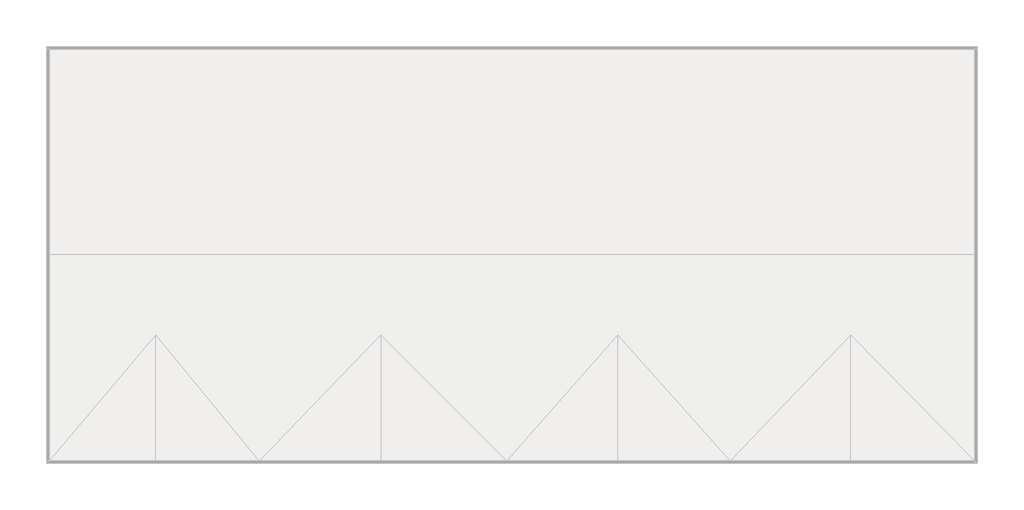
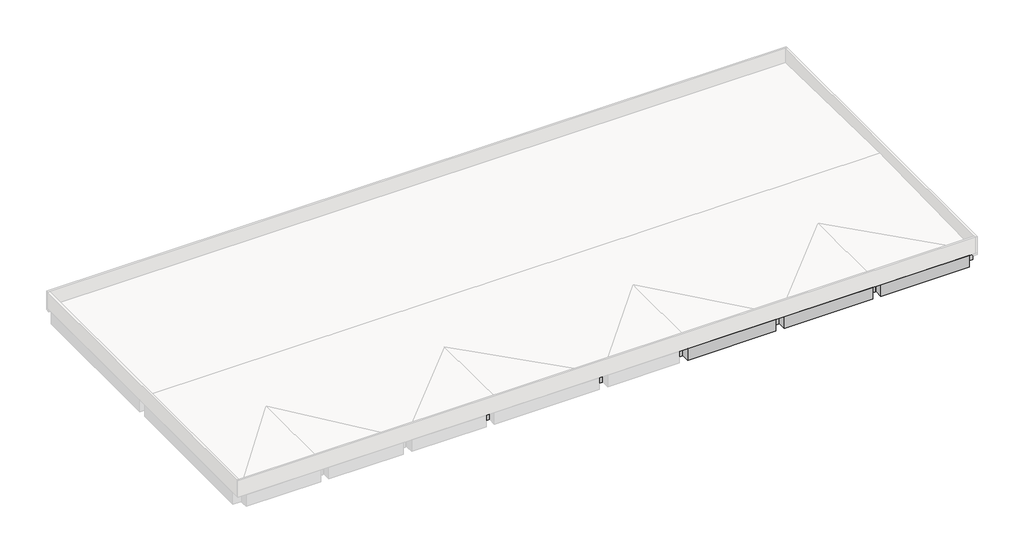
# One storey, part 2 of 2: 43 beams.
"""IFC4 building model written with IfcOpenShell, lengths in millimetres."""

import ifcopenshell
import ifcopenshell.guid

model = None  # the IFC model being written
_history = None  # IfcOwnerHistory: only IFC2X3 demands one
_inside = {}  # id of a spatial element -> (the spatial element, [elements in it])
_under = {}  # id of a project, library or spatial element -> (it, [spatial elements below it])
_declared = {}  # id of a project -> (the project, [libraries it declares])
_typed = {}  # id of a type object -> (the type object, [elements of that type])
_made_of = {}  # id of a material, layer set ... -> (it, [elements and type objects made of it])


def new_model(schema):
    """Start an empty IFC model of exactly this schema.

    Asked for "IFC4X3", IfcOpenShell would pick the latest addendum, in which some entities
    have other attributes; the version numbers below select the first issue.
    IFC2X3 requires an IfcOwnerHistory on every rooted entity: one is made here for all.
    """
    global model, _history
    if schema == "IFC4X3":
        model = ifcopenshell.file(schema_version=(4, 3, 0, 0))
    else:
        model = ifcopenshell.file(schema=schema)
    _inside.clear()
    _under.clear()
    _declared.clear()
    _typed.clear()
    _made_of.clear()
    _history = None
    if model.schema == "IFC2X3":
        org = make("IfcOrganization", Name="unknown")
        user = make(
            "IfcPersonAndOrganization",
            ThePerson=make("IfcPerson", FamilyName="unknown"),
            TheOrganization=org,
        )
        app = make(
            "IfcApplication",
            ApplicationDeveloper=org,
            Version="unknown",
            ApplicationFullName="unknown",
            ApplicationIdentifier="unknown",
        )
        _history = make(
            "IfcOwnerHistory",
            OwningUser=user,
            OwningApplication=app,
            ChangeAction="ADDED",
            CreationDate=0,
        )
    return model


def make(cls, **values):
    """One entity of the class cls with the attributes given. An attribute that is None is left unset."""
    return model.create_entity(
        cls, **{name: value for name, value in values.items() if value is not None}
    )


def rooted(cls, **values):
    """An entity with a GlobalId (a new one), such as an element, a storey or a relation."""
    return make(cls, GlobalId=ifcopenshell.guid.new(), OwnerHistory=_history, **values)


def si_unit(unit_type, name, prefix=None):
    """IfcSIUnit, for example si_unit("LENGTHUNIT", "METRE", prefix="MILLI")."""
    return make("IfcSIUnit", UnitType=unit_type, Prefix=prefix, Name=name)


def assignment(units):
    """IfcUnitAssignment: the units of a project."""
    return None if units is None else make("IfcUnitAssignment", Units=units)


def point(xyz):
    """IfcCartesianPoint."""
    return None if xyz is None else make("IfcCartesianPoint", Coordinates=xyz)


def direction(xyz):
    """IfcDirection."""
    return None if xyz is None else make("IfcDirection", DirectionRatios=xyz)


def frame(location, z_axis=None, x_axis=None):
    """IfcAxis2Placement3D, a coordinate frame: its origin and axes. An axis left out is left unset."""
    return make(
        "IfcAxis2Placement3D",
        Location=point(location),
        Axis=direction(z_axis),
        RefDirection=direction(x_axis),
    )


def origin():
    """The frame at (0, 0, 0) with its axes left unset."""
    return frame((0.0, 0.0, 0.0))


def place(relative_to, where):
    """IfcLocalPlacement: puts the frame where relative to a parent placement (None: the world)."""
    return make(
        "IfcLocalPlacement", PlacementRelTo=relative_to, RelativePlacement=where
    )


def context(
    kind, dimensions, precision=None, world=None, true_north=None, identifier=None
):
    """IfcGeometricRepresentationContext, for example the 3D "Model" context."""
    return make(
        "IfcGeometricRepresentationContext",
        ContextIdentifier=identifier,
        ContextType=kind,
        CoordinateSpaceDimension=dimensions,
        Precision=precision,
        WorldCoordinateSystem=world,
        TrueNorth=true_north,
    )


def project(units=None, contexts=None):
    """IfcProject with its units and contexts."""
    return rooted(
        "IfcProject",
        Name="project",
        RepresentationContexts=contexts,
        UnitsInContext=assignment(units),
    )


def spatial(cls, under=None, at=None, **own):
    """A site, building, storey or space (cls), placed at a placement, below another one or the project."""
    s = rooted(cls, ObjectPlacement=at, **own)
    if under is not None:
        _under.setdefault(under.id(), (under, []))[1].append(s)
    return s


def faces_of(points, faces, orient=None, outer=None):
    """IfcFace entities. A face is a list of loops; a loop is a list of indices into points, from 0.

    orient and outer hold one flag for each loop. By default every Orientation is true, the
    first loop of a face is its IfcFaceOuterBound and the others are IfcFaceBound.
    """
    made = []
    for i, loops in enumerate(faces):
        bounds = []
        for j, loop in enumerate(loops):
            is_outer = j == 0 if outer is None else outer[i][j]
            bounds.append(
                make(
                    "IfcFaceOuterBound" if is_outer else "IfcFaceBound",
                    Bound=make("IfcPolyLoop", Polygon=[points[k] for k in loop]),
                    Orientation=True if orient is None else orient[i][j],
                )
            )
        made.append(make("IfcFace", Bounds=bounds))
    return made


def faceted_brep(points, faces, orient=None, outer=None, voids=None):
    """IfcFacetedBrep: a solid bounded by flat faces; with voids (closed shells), ...WithVoids."""
    shared = [point(p) for p in points]
    hull = make("IfcClosedShell", CfsFaces=faces_of(shared, faces, orient, outer))
    if voids is None:
        return make("IfcFacetedBrep", Outer=hull)
    return make(
        "IfcFacetedBrepWithVoids",
        Outer=hull,
        Voids=[
            make(cls, CfsFaces=faces_of(shared, fs, o, b)) for cls, fs, o, b in voids
        ],
    )


def shape(context_of_items, identifier, shape_type, items):
    """IfcShapeRepresentation: the items that make up one representation, for example the "Body"."""
    return make(
        "IfcShapeRepresentation",
        ContextOfItems=context_of_items,
        RepresentationIdentifier=identifier,
        RepresentationType=shape_type,
        Items=items,
    )


def made_of(thing, what):
    """Note that an element or type object is made of a material, layer set ...; save() writes the relation."""
    if what is not None:
        _made_of.setdefault(what.id(), (what, []))[1].append(thing)
    return thing


def element(
    cls,
    number,
    at=None,
    inside=None,
    cuts=None,
    type_object=None,
    material=None,
    context=None,
    identifier="Body",
    shape_type=None,
    held_by="IfcProductDefinitionShape",
    body=None,
    shapes=None,
    **own,
):
    """One element of the class cls, such as IfcWall. Its Tag is "e" and its number.

    at: its placement. inside: the storey or other place that contains it. cuts: it is an
    opening in that element (IfcRelVoidsElement). A single representation is given by context,
    identifier, shape_type and body (its items); several are given by shapes. held_by: the class
    of the entity that holds the representations. save() writes the other relations.
    """
    e = rooted(cls, Tag="e%d" % number, ObjectPlacement=at, **own)
    if body is not None:
        shapes = [shape(context, identifier, shape_type, body)]
    if shapes is not None:
        e.Representation = make(held_by, Representations=shapes)
    if inside is not None:
        _inside.setdefault(inside.id(), (inside, []))[1].append(e)
    if cuts is not None:
        rooted(
            "IfcRelVoidsElement", RelatingBuildingElement=cuts, RelatedOpeningElement=e
        )
    if type_object is not None:
        _typed.setdefault(type_object.id(), (type_object, []))[1].append(e)
    return made_of(e, material)


def aggregate(whole, parts):
    """IfcRelAggregates: a whole, such as a stair, and the parts it consists of."""
    return rooted("IfcRelAggregates", RelatingObject=whole, RelatedObjects=parts)


def save(model, path):
    """Write the relations noted so far, then the file.

    IfcRelAggregates (storeys below a building ...), IfcRelContainedInSpatialStructure (elements
    in a storey), IfcRelDefinesByType, IfcRelAssociatesMaterial and IfcRelDeclares: one each for
    every whole, place, type object, material and project.
    """
    for whole, parts in _under.values():
        aggregate(whole, parts)
    for where, things in _inside.values():
        rooted(
            "IfcRelContainedInSpatialStructure",
            RelatedElements=things,
            RelatingStructure=where,
        )
    for kind, things in _typed.values():
        rooted("IfcRelDefinesByType", RelatedObjects=things, RelatingType=kind)
    for what, things in _made_of.values():
        rooted("IfcRelAssociatesMaterial", RelatedObjects=things, RelatingMaterial=what)
    for by, libraries in _declared.values():
        rooted("IfcRelDeclares", RelatingContext=by, RelatedDefinitions=libraries)
    model.write(path)


model = new_model("IFC4")

# Units and contexts
model_context = context("Model", 3, world=origin())
ifc_project = project(units=[si_unit("LENGTHUNIT", "METRE", prefix="MILLI")], contexts=[model_context])

# Site, building, storey
site = spatial("IfcSite", under=ifc_project)
building = spatial("IfcBuilding", under=site)
storey = spatial("IfcBuildingStorey", under=building, Name="TOC", Elevation=104550.0)

# Beams
placement = place(None, origin())
element("IfcBeam", 1, ObjectType="RC Beam_Rectangular : H_SB_AR S16_RC Beam-AG_600x900_RG9", at=placement, inside=storey, context=model_context, shape_type="Brep", body=[
    faceted_brep([(300.0, 4200.0, 104550.0), (300.0, 3600.0, 104550.0), (2800.0, 3600.0, 104550.0), (3200.0, 3600.0, 104550.0), (5700.0, 3600.0, 104550.0), (5700.0, 4200.0, 104550.0), (300.0, 3600.0, 104400.0), (300.0, 3600.0, 103650.0), (2800.0, 3600.0, 103650.0), (3200.0, 3600.0, 103650.0), (5700.0, 3600.0, 103650.0), (300.0, 4200.0, 103650.0), (5700.0, 4200.0, 103650.0)], [[[0, 1, 2, 3, 4, 5]], [[1, 6, 7, 8, 9, 10, 4, 3, 2]], [[7, 11, 12, 10, 9, 8]], [[11, 0, 5, 12]], [[1, 0, 11, 7, 6]], [[5, 4, 10, 12]]]),
])
element("IfcBeam", 2, ObjectType="RC Beam_Rectangular : H_SB_AR S16_RC Beam-AG_600x900_RG9", at=placement, inside=storey, context=model_context, shape_type="Brep", body=[
    faceted_brep([(6300.0, 4200.0, 104550.0), (6300.0, 3600.0, 104550.0), (8800.0, 3600.0, 104550.0), (9200.0, 3600.0, 104550.0), (11700.0, 3600.0, 104550.0), (11700.0, 4200.0, 104550.0), (6300.0, 3600.0, 103650.0), (8800.0, 3600.0, 103650.0), (9200.0, 3600.0, 103650.0), (11700.0, 3600.0, 103650.0), (6300.0, 4200.0, 103650.0), (11700.0, 4200.0, 103650.0)], [[[0, 1, 2, 3, 4, 5]], [[1, 6, 7, 8, 9, 4, 3, 2]], [[6, 10, 11, 9, 8, 7]], [[10, 0, 5, 11]], [[1, 0, 10, 6]], [[5, 4, 9, 11]]]),
])
element("IfcBeam", 3, ObjectType="RC Beam_Rectangular : H_SB_AR S16_RC Beam-AG_600x900_RG9", at=placement, inside=storey, context=model_context, shape_type="Brep", body=[
    faceted_brep([(12300.0, 4200.0, 104550.0), (12300.0, 3600.0, 104550.0), (14800.0, 3600.0, 104550.0), (15200.0, 3600.0, 104550.0), (17700.0, 3600.0, 104550.0), (17700.0, 4200.0, 104550.0), (12300.0, 3600.0, 103650.0), (14800.0, 3600.0, 103650.0), (15200.0, 3600.0, 103650.0), (17700.0, 3600.0, 103650.0), (17700.0, 3600.0, 104400.0), (12300.0, 4200.0, 103650.0), (17700.0, 4200.0, 103650.0)], [[[0, 1, 2, 3, 4, 5]], [[1, 6, 7, 8, 9, 10, 4, 3, 2]], [[6, 11, 12, 9, 8, 7]], [[11, 0, 5, 12]], [[1, 0, 11, 6]], [[5, 4, 10, 9, 12]]]),
])
element("IfcBeam", 4, ObjectType="RC Beam_Rectangular : H_SB_AR S16_RC Beam-AG_600x900_RG9", at=placement, inside=storey, context=model_context, shape_type="Brep", body=[
    faceted_brep([(18300.0, 4200.0, 104550.0), (18300.0, 3600.0, 104550.0), (21800.0, 3600.0, 104550.0), (22400.0, 3600.0, 104550.0), (25900.0, 3600.0, 104550.0), (25900.0, 4200.0, 104550.0), (18300.0, 3600.0, 104400.0), (18300.0, 3600.0, 103650.0), (21800.0, 3600.0, 103650.0), (22400.0, 3600.0, 103650.0), (25900.0, 3600.0, 103650.0), (18300.0, 4200.0, 103650.0), (25900.0, 4200.0, 103650.0)], [[[0, 1, 2, 3, 4, 5]], [[1, 6, 7, 8, 9, 10, 4, 3, 2]], [[7, 11, 12, 10, 9, 8]], [[11, 0, 5, 12]], [[7, 6, 1, 0, 11]], [[5, 4, 10, 12]]]),
])
element("IfcBeam", 5, ObjectType="RC Beam_Rectangular : H_SB_AR S16_RC Beam-AG_600x900_RG9", at=placement, inside=storey, context=model_context, shape_type="Brep", body=[
    faceted_brep([(31700.0, 3600.0, 104550.0), (31700.0, 4200.0, 104550.0), (26500.0, 4200.0, 104550.0), (26500.0, 3600.0, 104550.0), (28800.0, 3600.0, 104550.0), (29400.0, 3600.0, 104550.0), (31700.0, 3600.0, 103650.0), (26500.0, 3600.0, 103650.0), (28800.0, 3600.0, 103650.0), (29400.0, 3600.0, 103650.0), (31700.0, 4200.0, 103650.0), (26500.0, 4200.0, 103650.0)], [[[0, 1, 2, 3, 4, 5]], [[6, 0, 5, 4, 3, 7, 8, 9]], [[10, 6, 9, 8, 7, 11]], [[1, 10, 11, 2]], [[1, 0, 6, 10]], [[3, 2, 11, 7]]]),
])
element("IfcBeam", 6, ObjectType="RC Beam_Rectangular : H_SB_AR S16_RC Beam-AG_600x900_RG9", at=placement, inside=storey, context=model_context, shape_type="Brep", body=[
    faceted_brep([(38700.0, 3600.0, 104550.0), (38700.0, 4200.0, 104550.0), (32300.0, 4200.0, 104550.0), (32300.0, 3600.0, 104550.0), (35200.0, 3600.0, 104550.0), (35800.0, 3600.0, 104550.0), (38700.0, 3600.0, 103650.0), (32300.0, 3600.0, 103650.0), (35200.0, 3600.0, 103650.0), (35800.0, 3600.0, 103650.0), (38700.0, 4200.0, 103650.0), (32300.0, 4200.0, 103650.0)], [[[0, 1, 2, 3, 4, 5]], [[6, 0, 5, 4, 3, 7, 8, 9]], [[10, 6, 9, 8, 7, 11]], [[1, 10, 11, 2]], [[1, 0, 6, 10]], [[3, 2, 11, 7]]]),
])
element("IfcBeam", 7, ObjectType="RC Beam_Rectangular : H_SB_AR S16_RC Beam-AG_600x900_RG9", at=placement, inside=storey, context=model_context, shape_type="Brep", body=[
    faceted_brep([(45700.0, 3600.0, 104550.0), (45700.0, 4200.0, 104550.0), (39300.0, 4200.0, 104550.0), (39300.0, 3600.0, 104550.0), (42200.0, 3600.0, 104550.0), (42800.0, 3600.0, 104550.0), (45700.0, 3600.0, 103650.0), (39300.0, 3600.0, 103650.0), (42200.0, 3600.0, 103650.0), (42800.0, 3600.0, 103650.0), (45700.0, 4200.0, 103650.0), (39300.0, 4200.0, 103650.0)], [[[0, 1, 2, 3, 4, 5]], [[6, 0, 5, 4, 3, 7, 8, 9]], [[10, 6, 9, 8, 7, 11]], [[1, 10, 11, 2]], [[1, 0, 6, 10]], [[3, 2, 11, 7]]]),
])
element("IfcBeam", 8, ObjectType="RC Beam_Rectangular : H_SB_AR S16_RC Beam-AG_600x900_RG9", at=placement, inside=storey, context=model_context, shape_type="Brep", body=[
    faceted_brep([(52700.0, 3600.0, 104550.0), (52700.0, 4200.0, 104550.0), (46300.0, 4200.0, 104550.0), (46300.0, 3600.0, 104550.0), (46600.0, 3600.0, 104550.0), (47200.0, 3600.0, 104550.0), (52700.0, 3600.0, 103650.0), (52700.0, 3600.0, 104400.0), (46300.0, 3600.0, 103650.0), (46600.0, 3600.0, 103650.0), (47200.0, 3600.0, 103650.0), (52700.0, 4200.0, 103650.0), (46300.0, 4200.0, 103650.0)], [[[0, 1, 2, 3, 4, 5]], [[6, 7, 0, 5, 4, 3, 8, 9, 10]], [[11, 6, 10, 9, 8, 12]], [[1, 11, 12, 2]], [[1, 0, 7, 6, 11]], [[3, 2, 12, 8]]]),
])
element("IfcBeam", 9, ObjectType="RC Beam_Rectangular : H_SB_AR S16_RC Beam-AG_600x900_RG9", at=placement, inside=storey, context=model_context, shape_type="Brep", body=[
    faceted_brep([(32300.0, -19200.0, 104550.0), (32300.0, -19800.0, 104550.0), (38700.0, -19800.0, 104550.0), (38700.0, -19200.0, 104550.0), (35800.0, -19200.0, 104550.0), (35200.0, -19200.0, 104550.0), (32300.0, -19800.0, 103650.0), (38700.0, -19800.0, 103650.0), (32300.0, -19200.0, 103650.0), (35200.0, -19200.0, 103650.0), (35800.0, -19200.0, 103650.0), (38700.0, -19200.0, 103650.0)], [[[0, 1, 2, 3, 4, 5]], [[1, 6, 7, 2]], [[6, 8, 9, 10, 11, 7]], [[8, 0, 5, 4, 3, 11, 10, 9]], [[1, 0, 8, 6]], [[3, 2, 7, 11]]]),
])
element("IfcBeam", 10, ObjectType="RC Beam_Rectangular : H_SB_AR S16_RC Beam-AG_600x900_RG9", at=placement, inside=storey, context=model_context, shape_type="Brep", body=[
    faceted_brep([(39300.0, -19200.0, 104550.0), (39300.0, -19800.0, 104550.0), (45700.0, -19800.0, 104550.0), (45700.0, -19200.0, 104550.0), (42800.0, -19200.0, 104550.0), (42200.0, -19200.0, 104550.0), (39300.0, -19800.0, 103650.0), (45700.0, -19800.0, 103650.0), (39300.0, -19200.0, 103650.0), (42200.0, -19200.0, 103650.0), (42800.0, -19200.0, 103650.0), (45700.0, -19200.0, 103650.0)], [[[0, 1, 2, 3, 4, 5]], [[1, 6, 7, 2]], [[6, 8, 9, 10, 11, 7]], [[8, 0, 5, 4, 3, 11, 10, 9]], [[1, 0, 8, 6]], [[3, 2, 7, 11]]]),
])
element("IfcBeam", 11, ObjectType="RC Beam_Rectangular : H_SB_AR S16_RC Beam-AG_600x900_RG9", at=placement, inside=storey, context=model_context, shape_type="Brep", body=[
    faceted_brep([(46300.0, -19200.0, 104550.0), (46300.0, -19800.0, 104550.0), (52700.0, -19800.0, 104550.0), (52700.0, -19200.0, 104550.0), (49800.0, -19200.0, 104550.0), (49200.0, -19200.0, 104550.0), (46300.0, -19800.0, 103650.0), (52700.0, -19800.0, 103650.0), (46300.0, -19200.0, 103650.0), (49200.0, -19200.0, 103650.0), (49800.0, -19200.0, 103650.0), (52700.0, -19200.0, 103650.0), (52700.0, -19350.0, 103650.0), (52700.0, -19200.0, 104400.0)], [[[0, 1, 2, 3, 4, 5]], [[1, 6, 7, 2]], [[6, 8, 9, 10, 11, 12, 7]], [[8, 0, 5, 4, 3, 13, 11, 10, 9]], [[1, 0, 8, 6]], [[3, 2, 7, 12, 11, 13]]]),
])
element("IfcBeam", 12, ObjectType="RC Beam_Rectangular : H_SB_AR S16_RC Beam-AG_600x900_RG7", at=placement, inside=storey, context=model_context, shape_type="Brep", body=[
    faceted_brep([(53300.0, 3600.0, 104550.0), (52700.0, 3600.0, 104550.0), (52700.0, -11400.0, 104550.0), (53300.0, -11400.0, 104550.0), (52700.0, 3600.0, 104400.0), (52700.0, 3600.0, 103650.0), (52700.0, -11400.0, 103650.0), (52700.0, -11400.0, 104400.0), (52850.0, 3600.0, 103650.0), (53300.0, 3600.0, 103650.0), (53300.0, -11400.0, 103650.0)], [[[0, 1, 2, 3]], [[1, 4, 5, 6, 7, 2]], [[5, 8, 9, 10, 6]], [[3, 10, 9, 0]], [[0, 9, 8, 5, 4, 1]], [[3, 2, 7, 6, 10]]]),
])
element("IfcBeam", 13, ObjectType="RC Beam_Rectangular : H_SB_AR S16_RC Beam-AG_600x900_RG8", at=placement, inside=storey, context=model_context, shape_type="Brep", body=[
    faceted_brep([(53300.0, -12000.0, 104550.0), (52700.0, -12000.0, 104550.0), (52700.0, -19200.0, 104550.0), (53300.0, -19200.0, 104550.0), (52700.0, -19200.0, 103650.0), (52700.0, -19200.0, 104400.0), (52700.0, -12000.0, 104400.0), (52700.0, -12000.0, 103650.0), (53300.0, -19200.0, 103650.0), (53300.0, -12000.0, 103650.0)], [[[0, 1, 2, 3]], [[4, 5, 2, 1, 6, 7]], [[8, 4, 7, 9]], [[3, 8, 9, 0]], [[2, 5, 4, 8, 3]], [[0, 9, 7, 6, 1]]]),
])
element("IfcBeam", 14, ObjectType="RC Beam_Rectangular : H_SB_AR S16_RC Beam-AG_600x900_RG5", at=placement, inside=storey, context=model_context, shape_type="Brep", body=[
    faceted_brep([(52700.0, -12000.0, 104550.0), (52700.0, -11400.0, 104550.0), (47200.0, -11400.0, 104550.0), (46600.0, -11400.0, 104550.0), (46300.0, -11400.0, 104550.0), (46300.0, -12000.0, 104550.0), (49200.0, -12000.0, 104550.0), (49800.0, -12000.0, 104550.0), (52700.0, -11400.0, 104400.0), (52700.0, -11400.0, 103650.0), (47200.0, -11400.0, 103650.0), (46600.0, -11400.0, 103650.0), (46300.0, -11400.0, 103650.0), (52700.0, -11600.0, 103650.0), (52700.0, -12000.0, 103650.0), (49800.0, -12000.0, 103650.0), (49200.0, -12000.0, 103650.0), (46300.0, -12000.0, 103650.0), (46300.0, -11600.0, 103650.0), (52700.0, -12000.0, 104400.0)], [[[0, 1, 2, 3, 4, 5, 6, 7]], [[1, 8, 9, 10, 11, 12, 4, 3, 2]], [[9, 13, 14, 15, 16, 17, 18, 12, 11, 10]], [[5, 17, 16, 15, 14, 19, 0, 7, 6]], [[0, 19, 14, 13, 9, 8, 1]], [[5, 4, 12, 18, 17]]]),
])
element("IfcBeam", 15, ObjectType="RC Beam_Rectangular : H_SB_AR S16_RC Beam-AG_600x900_RG5", at=placement, inside=storey, context=model_context, shape_type="Brep", body=[
    faceted_brep([(39300.0, -11400.0, 104550.0), (39300.0, -12000.0, 104550.0), (42200.0, -12000.0, 104550.0), (42800.0, -12000.0, 104550.0), (45700.0, -12000.0, 104550.0), (45700.0, -11400.0, 104550.0), (42800.0, -11400.0, 104550.0), (42200.0, -11400.0, 104550.0), (39300.0, -11400.0, 103650.0), (45700.0, -11400.0, 103650.0), (45000.0, -11400.0, 103650.0), (43500.0, -11400.0, 103650.0), (43300.0, -11400.0, 103650.0), (42800.0, -11400.0, 103650.0), (42200.0, -11400.0, 103650.0), (39300.0, -12000.0, 103650.0), (39300.0, -11600.0, 103650.0), (45700.0, -11600.0, 103650.0), (45700.0, -12000.0, 103650.0), (45200.0, -12000.0, 103650.0), (45000.0, -12000.0, 103650.0), (43500.0, -12000.0, 103650.0), (43300.0, -12000.0, 103650.0), (42800.0, -12000.0, 103650.0), (42200.0, -12000.0, 103650.0), (42100.0, -12000.0, 103650.0)], [[[0, 1, 2, 3, 4, 5, 6, 7]], [[8, 0, 7, 6, 5, 9, 10, 11, 12, 13, 14]], [[15, 16, 8, 14, 13, 12, 11, 10, 9, 17, 18, 19, 20, 21, 22, 23, 24, 25]], [[1, 15, 25, 24, 23, 22, 21, 20, 19, 18, 4, 3, 2]], [[1, 0, 8, 16, 15]], [[5, 4, 18, 17, 9]]]),
])
element("IfcBeam", 16, ObjectType="RC Beam_Rectangular : H_SB_AR S16_RC Beam-AG_600x900_RG5", at=placement, inside=storey, context=model_context, shape_type="Brep", body=[
    faceted_brep([(32300.0, -11400.0, 104550.0), (32300.0, -12000.0, 104550.0), (35200.0, -12000.0, 104550.0), (35800.0, -12000.0, 104550.0), (38700.0, -12000.0, 104550.0), (38700.0, -11400.0, 104550.0), (35800.0, -11400.0, 104550.0), (35200.0, -11400.0, 104550.0), (32300.0, -11400.0, 103650.0), (38700.0, -11400.0, 103650.0), (36700.0, -11400.0, 103650.0), (35800.0, -11400.0, 103650.0), (35200.0, -11400.0, 103650.0), (32300.0, -12000.0, 103650.0), (32300.0, -11600.0, 103650.0), (38700.0, -12000.0, 103650.0), (36700.0, -12000.0, 103650.0), (36500.0, -12000.0, 103650.0), (35800.0, -12000.0, 103650.0), (35200.0, -12000.0, 103650.0)], [[[0, 1, 2, 3, 4, 5, 6, 7]], [[8, 0, 7, 6, 5, 9, 10, 11, 12]], [[13, 14, 8, 12, 11, 10, 9, 15, 16, 17, 18, 19]], [[1, 13, 19, 18, 17, 16, 15, 4, 3, 2]], [[1, 0, 8, 14, 13]], [[5, 4, 15, 9]]]),
])
element("IfcBeam", 17, ObjectType="RC Beam_Rectangular : H_SB_AR S16_RC Beam-AG_600x900_RG5", at=placement, inside=storey, context=model_context, shape_type="Brep", body=[
    faceted_brep([(26500.0, -11400.0, 104550.0), (26500.0, -12000.0, 104550.0), (28800.0, -12000.0, 104550.0), (29400.0, -12000.0, 104550.0), (31700.0, -12000.0, 104550.0), (31700.0, -11400.0, 104550.0), (29400.0, -11400.0, 104550.0), (28800.0, -11400.0, 104550.0), (26500.0, -11400.0, 103650.0), (31700.0, -11400.0, 103650.0), (29400.0, -11400.0, 103650.0), (28800.0, -11400.0, 103650.0), (26500.0, -12000.0, 103650.0), (26500.0, -11600.0, 103650.0), (31700.0, -11600.0, 103650.0), (31700.0, -12000.0, 103650.0), (29400.0, -12000.0, 103650.0), (28800.0, -12000.0, 103650.0), (28700.0, -12000.0, 103650.0), (28500.0, -12000.0, 103650.0)], [[[0, 1, 2, 3, 4, 5, 6, 7]], [[8, 0, 7, 6, 5, 9, 10, 11]], [[12, 13, 8, 11, 10, 9, 14, 15, 16, 17, 18, 19]], [[1, 12, 19, 18, 17, 16, 15, 4, 3, 2]], [[1, 0, 8, 13, 12]], [[5, 4, 15, 14, 9]]]),
])
element("IfcBeam", 18, ObjectType="RC Beam_Rectangular : H_SB_AR S16_RC Beam-AG_600x900_RG5A", at=placement, inside=storey, context=model_context, shape_type="Brep", body=[
    faceted_brep([(18300.0, -11400.0, 104550.0), (18300.0, -12000.0, 104550.0), (21800.0, -12000.0, 104550.0), (22400.0, -12000.0, 104550.0), (25900.0, -12000.0, 104550.0), (25900.0, -11400.0, 104550.0), (22400.0, -11400.0, 104550.0), (21800.0, -11400.0, 104550.0), (18300.0, -11400.0, 103650.0), (18300.0, -11400.0, 104400.0), (25900.0, -11400.0, 103650.0), (22400.0, -11400.0, 103650.0), (21800.0, -11400.0, 103650.0), (18300.0, -12000.0, 103650.0), (18300.0, -11600.0, 103650.0), (25900.0, -11600.0, 103650.0), (25900.0, -12000.0, 103650.0), (22400.0, -12000.0, 103650.0), (21800.0, -12000.0, 103650.0), (18300.0, -12000.0, 104400.0)], [[[0, 1, 2, 3, 4, 5, 6, 7]], [[8, 9, 0, 7, 6, 5, 10, 11, 12]], [[13, 14, 8, 12, 11, 10, 15, 16, 17, 18]], [[1, 19, 13, 18, 17, 16, 4, 3, 2]], [[1, 0, 9, 8, 14, 13, 19]], [[5, 4, 16, 15, 10]]]),
])
element("IfcBeam", 19, ObjectType="RC Beam_Rectangular : H_SB_AR S16_RC Beam-AG_600x900_RG4", at=placement, inside=storey, context=model_context, shape_type="Brep", body=[
    faceted_brep([(6300.0, -7500.0, 104550.0), (6300.0, -8100.0, 104550.0), (8800.0, -8100.0, 104550.0), (9200.0, -8100.0, 104550.0), (11700.0, -8100.0, 104550.0), (11700.0, -7500.0, 104550.0), (9200.0, -7500.0, 104550.0), (8800.0, -7500.0, 104550.0), (6300.0, -8100.0, 103650.0), (8800.0, -8100.0, 103650.0), (9200.0, -8100.0, 103650.0), (11700.0, -8100.0, 103650.0), (6300.0, -7500.0, 103650.0), (8800.0, -7500.0, 103650.0), (9200.0, -7500.0, 103650.0), (11700.0, -7500.0, 103650.0)], [[[0, 1, 2, 3, 4, 5, 6, 7]], [[1, 8, 9, 10, 11, 4, 3, 2]], [[8, 12, 13, 14, 15, 11, 10, 9]], [[12, 0, 7, 6, 5, 15, 14, 13]], [[1, 0, 12, 8]], [[5, 4, 11, 15]]]),
])
element("IfcBeam", 20, ObjectType="RC Beam_Rectangular : H_SB_AR S16_RC Beam-AG_600x900_RG4", at=placement, inside=storey, context=model_context, shape_type="Brep", body=[
    faceted_brep([(12300.0, -7500.0, 104550.0), (12300.0, -8100.0, 104550.0), (14800.0, -8100.0, 104550.0), (15200.0, -8100.0, 104550.0), (17700.0, -8100.0, 104550.0), (17700.0, -7500.0, 104550.0), (15200.0, -7500.0, 104550.0), (14800.0, -7500.0, 104550.0), (12300.0, -8100.0, 103650.0), (14800.0, -8100.0, 103650.0), (15200.0, -8100.0, 103650.0), (17700.0, -8100.0, 103650.0), (17700.0, -8100.0, 104400.0), (12300.0, -7500.0, 103650.0), (14800.0, -7500.0, 103650.0), (15200.0, -7500.0, 103650.0), (17700.0, -7500.0, 103650.0), (17700.0, -7900.0, 103650.0), (17700.0, -7500.0, 104400.0)], [[[0, 1, 2, 3, 4, 5, 6, 7]], [[1, 8, 9, 10, 11, 12, 4, 3, 2]], [[8, 13, 14, 15, 16, 17, 11, 10, 9]], [[13, 0, 7, 6, 5, 18, 16, 15, 14]], [[1, 0, 13, 8]], [[5, 4, 12, 11, 17, 16, 18]]]),
])
element("IfcBeam", 21, ObjectType="RC Beam_Rectangular : H_SB_AR S16_RC Beam-AG_600x900_RG1A", at=placement, inside=storey, context=model_context, shape_type="Brep", body=[
    faceted_brep([(18300.0, -8100.0, 104550.0), (17700.0, -8100.0, 104550.0), (17700.0, -19200.0, 104550.0), (18300.0, -19200.0, 104550.0), (18300.0, -12000.0, 104550.0), (18300.0, -11400.0, 104550.0), (18300.0, -19200.0, 104400.0), (18300.0, -19200.0, 103650.0), (18300.0, -12000.0, 103650.0), (18300.0, -11400.0, 103650.0), (18300.0, -8100.0, 103650.0), (17700.0, -19200.0, 103650.0), (17700.0, -8100.0, 103650.0), (18100.0, -8100.0, 103650.0), (18100.0, -19200.0, 103650.0), (17700.0, -19200.0, 104400.0), (17700.0, -8100.0, 104400.0)], [[[0, 1, 2, 3, 4, 5]], [[3, 6, 7, 8, 9, 10, 0, 5, 4]], [[11, 12, 13, 10, 9, 8, 7, 14]], [[11, 15, 2, 1, 16, 12]], [[2, 15, 11, 14, 7, 6, 3]], [[0, 10, 13, 12, 16, 1]]]),
])
element("IfcBeam", 22, ObjectType="RC Beam_Rectangular : H_SB_AR S16_RC Beam-AG_600x900_RG1A", at=placement, inside=storey, context=model_context, shape_type="Brep", body=[
    faceted_brep([(18300.0, 3600.0, 104550.0), (17700.0, 3600.0, 104550.0), (17700.0, -7500.0, 104550.0), (18300.0, -7500.0, 104550.0), (18300.0, -7500.0, 103650.0), (18300.0, 3600.0, 103650.0), (18300.0, 3600.0, 104400.0), (17700.0, -7500.0, 103650.0), (17700.0, 3600.0, 103650.0), (18100.0, 3600.0, 103650.0), (18100.0, -7500.0, 103650.0), (17700.0, -7500.0, 104400.0), (17700.0, 3600.0, 104400.0)], [[[0, 1, 2, 3]], [[3, 4, 5, 6, 0]], [[7, 8, 9, 5, 4, 10]], [[7, 11, 2, 1, 12, 8]], [[2, 11, 7, 10, 4, 3]], [[0, 6, 5, 9, 8, 12, 1]]]),
])
element("IfcBeam", 23, ObjectType="RC Beam_Rectangular : H_SB_AR S16_RC Beam-AG_400x900_RG1", at=placement, inside=storey, context=model_context, shape_type="Brep", body=[
    faceted_brep([(12200.0, 3600.0, 104550.0), (11800.0, 3600.0, 104550.0), (11800.0, -7500.0, 104550.0), (12200.0, -7500.0, 104550.0), (12200.0, -7500.0, 104400.0), (12200.0, -7500.0, 103650.0), (12200.0, 3600.0, 103650.0), (12200.0, 3600.0, 104400.0), (11800.0, 3600.0, 103650.0), (11800.0, -7500.0, 103650.0), (11800.0, -7500.0, 104400.0), (11800.0, 3600.0, 104400.0)], [[[0, 1, 2, 3]], [[3, 4, 5, 6, 7, 0]], [[8, 6, 5, 9]], [[9, 10, 2, 1, 11, 8]], [[2, 10, 9, 5, 4, 3]], [[0, 7, 6, 8, 11, 1]]]),
])
element("IfcBeam", 24, ObjectType="RC Beam_Rectangular : H_SB_AR S16_RC Beam-AG_400x900_RB1", at=placement, inside=storey, context=model_context, shape_type="Brep", body=[
    faceted_brep([(9200.0, 3600.0, 104550.0), (8800.0, 3600.0, 104550.0), (8800.0, -7500.0, 104550.0), (9200.0, -7500.0, 104550.0), (8800.0, 3600.0, 104400.0), (8800.0, 3600.0, 103650.0), (8800.0, -7500.0, 103650.0), (8800.0, -7500.0, 104400.0), (9200.0, 3600.0, 103650.0), (9200.0, -7500.0, 103650.0), (9200.0, 3600.0, 104400.0), (9200.0, -7500.0, 104400.0)], [[[0, 1, 2, 3]], [[1, 4, 5, 6, 7, 2]], [[5, 8, 9, 6]], [[8, 10, 0, 3, 11, 9]], [[1, 0, 10, 8, 5, 4]], [[3, 2, 7, 6, 9, 11]]]),
])
element("IfcBeam", 25, ObjectType="RC Beam_Rectangular : H_SB_AR S16_RC Beam-AG_400x900_RB1", at=placement, inside=storey, context=model_context, shape_type="Brep", body=[
    faceted_brep([(15200.0, 3600.0, 104550.0), (14800.0, 3600.0, 104550.0), (14800.0, -7500.0, 104550.0), (15200.0, -7500.0, 104550.0), (14800.0, 3600.0, 104400.0), (14800.0, 3600.0, 103650.0), (14800.0, -7500.0, 103650.0), (14800.0, -7500.0, 104400.0), (15200.0, 3600.0, 103650.0), (15200.0, -7500.0, 103650.0), (15200.0, 3600.0, 104400.0), (15200.0, -7500.0, 104400.0)], [[[0, 1, 2, 3]], [[1, 4, 5, 6, 7, 2]], [[5, 8, 9, 6]], [[8, 10, 0, 3, 11, 9]], [[1, 0, 10, 8, 5, 4]], [[3, 2, 7, 6, 9, 11]]]),
])
element("IfcBeam", 26, ObjectType="RC Beam_Rectangular : H_SB_AR S16_RC Beam-AG_500x900_RG2", at=placement, inside=storey, context=model_context, shape_type="Brep", body=[
    faceted_brep([(26450.0, 3600.0, 104550.0), (25950.0, 3600.0, 104550.0), (25950.0, -11400.0, 104550.0), (26450.0, -11400.0, 104550.0), (25950.0, 3600.0, 104400.0), (25950.0, 3600.0, 103650.0), (25950.0, -11400.0, 103650.0), (25950.0, -11400.0, 104400.0), (26450.0, 3600.0, 103650.0), (26450.0, -11400.0, 103650.0), (26450.0, -11400.0, 104400.0), (26450.0, 3600.0, 104400.0)], [[[0, 1, 2, 3]], [[1, 4, 5, 6, 7, 2]], [[5, 8, 9, 6]], [[3, 10, 9, 8, 11, 0]], [[9, 10, 3, 2, 7, 6]], [[0, 11, 8, 5, 4, 1]]]),
])
element("IfcBeam", 27, ObjectType="RC Beam_Rectangular : H_SB_AR S16_RC Beam-AG_500x900_RG3", at=placement, inside=storey, context=model_context, shape_type="Brep", body=[
    faceted_brep([(25950.0, -19200.0, 104550.0), (26450.0, -19200.0, 104550.0), (26450.0, -12000.0, 104550.0), (25950.0, -12000.0, 104550.0), (25950.0, -19200.0, 103650.0), (25950.0, -19200.0, 104400.0), (25950.0, -12000.0, 104400.0), (25950.0, -12000.0, 103650.0), (26450.0, -19200.0, 103650.0), (26300.0, -19200.0, 103650.0), (26300.0, -12000.0, 103650.0), (26450.0, -12000.0, 103650.0), (26450.0, -12000.0, 104400.0), (26450.0, -19200.0, 104400.0)], [[[0, 1, 2, 3]], [[4, 5, 0, 3, 6, 7]], [[8, 9, 4, 7, 10, 11]], [[11, 12, 2, 1, 13, 8]], [[0, 5, 4, 9, 8, 13, 1]], [[2, 12, 11, 10, 7, 6, 3]]]),
])
element("IfcBeam", 28, ObjectType="RC Beam_Rectangular : H_SB_AR S16_RC Beam-AG_500x900_RG2", at=placement, inside=storey, context=model_context, shape_type="Brep", body=[
    faceted_brep([(32250.0, 3600.0, 104550.0), (31750.0, 3600.0, 104550.0), (31750.0, -11400.0, 104550.0), (32250.0, -11400.0, 104550.0), (31750.0, 3600.0, 104400.0), (31750.0, 3600.0, 103650.0), (31750.0, -11400.0, 103650.0), (31750.0, -11400.0, 104400.0), (32250.0, 3600.0, 103650.0), (32250.0, -11400.0, 103650.0), (32250.0, -11400.0, 104400.0), (32250.0, 3600.0, 104400.0)], [[[0, 1, 2, 3]], [[1, 4, 5, 6, 7, 2]], [[5, 8, 9, 6]], [[3, 10, 9, 8, 11, 0]], [[9, 10, 3, 2, 7, 6]], [[0, 11, 8, 5, 4, 1]]]),
])
element("IfcBeam", 29, ObjectType="RC Beam_Rectangular : H_SB_AR S16_RC Beam-AG_500x900_RG3", at=placement, inside=storey, context=model_context, shape_type="Brep", body=[
    faceted_brep([(31750.0, -19200.0, 104550.0), (32250.0, -19200.0, 104550.0), (32250.0, -12000.0, 104550.0), (31750.0, -12000.0, 104550.0), (31750.0, -19200.0, 103650.0), (31750.0, -19200.0, 104400.0), (31750.0, -12000.0, 104400.0), (31750.0, -12000.0, 103650.0), (32250.0, -19200.0, 103650.0), (31900.0, -19200.0, 103650.0), (31900.0, -12000.0, 103650.0), (32250.0, -12000.0, 103650.0), (32250.0, -12000.0, 104400.0), (32250.0, -19200.0, 104400.0)], [[[0, 1, 2, 3]], [[4, 5, 0, 3, 6, 7]], [[8, 9, 4, 7, 10, 11]], [[11, 12, 2, 1, 13, 8]], [[0, 5, 4, 9, 8, 13, 1]], [[2, 12, 11, 10, 7, 6, 3]]]),
])
element("IfcBeam", 30, ObjectType="RC Beam_Rectangular : H_SB_AR S16_RC Beam-AG_500x900_RG2", at=placement, inside=storey, context=model_context, shape_type="Brep", body=[
    faceted_brep([(39250.0, 3600.0, 104550.0), (38750.0, 3600.0, 104550.0), (38750.0, -11400.0, 104550.0), (39250.0, -11400.0, 104550.0), (38750.0, 3600.0, 104400.0), (38750.0, 3600.0, 103650.0), (38750.0, -9150.0, 103650.0), (38750.0, -9350.0, 103650.0), (38750.0, -11400.0, 103650.0), (38750.0, -11400.0, 104400.0), (39250.0, 3600.0, 103650.0), (39250.0, -9150.0, 103650.0), (39250.0, -9350.0, 103650.0), (39250.0, -11400.0, 103650.0), (39250.0, -11400.0, 104400.0), (39250.0, 3600.0, 104400.0)], [[[0, 1, 2, 3]], [[1, 4, 5, 6, 7, 8, 9, 2]], [[5, 10, 11, 12, 13, 8, 7, 6]], [[3, 14, 13, 12, 11, 10, 15, 0]], [[13, 14, 3, 2, 9, 8]], [[0, 15, 10, 5, 4, 1]]]),
])
element("IfcBeam", 31, ObjectType="RC Beam_Rectangular : H_SB_AR S16_RC Beam-AG_500x900_RG3", at=placement, inside=storey, context=model_context, shape_type="Brep", body=[
    faceted_brep([(38750.0, -19200.0, 104550.0), (39250.0, -19200.0, 104550.0), (39250.0, -12000.0, 104550.0), (38750.0, -12000.0, 104550.0), (38750.0, -19200.0, 103650.0), (38750.0, -19200.0, 104400.0), (38750.0, -12000.0, 104400.0), (38750.0, -12000.0, 103650.0), (39250.0, -19200.0, 103650.0), (38900.0, -19200.0, 103650.0), (38900.0, -12000.0, 103650.0), (39250.0, -12000.0, 103650.0), (39250.0, -15150.0, 103650.0), (39250.0, -15350.0, 103650.0), (39250.0, -12000.0, 104400.0), (39250.0, -19200.0, 104400.0)], [[[0, 1, 2, 3]], [[4, 5, 0, 3, 6, 7]], [[8, 9, 4, 7, 10, 11, 12, 13]], [[11, 14, 2, 1, 15, 8, 13, 12]], [[0, 5, 4, 9, 8, 15, 1]], [[2, 14, 11, 10, 7, 6, 3]]]),
])
element("IfcBeam", 32, ObjectType="RC Beam_Rectangular : H_SB_AR S16_RC Beam-AG_500x900_RG2", at=placement, inside=storey, context=model_context, shape_type="Brep", body=[
    faceted_brep([(46250.0, 3600.0, 104550.0), (45750.0, 3600.0, 104550.0), (45750.0, -11400.0, 104550.0), (46250.0, -11400.0, 104550.0), (45750.0, 3600.0, 104400.0), (45750.0, 3600.0, 103650.0), (45750.0, 900.0, 103650.0), (45750.0, 700.0, 103650.0), (45750.0, -9150.0, 103650.0), (45750.0, -9350.0, 103650.0), (45750.0, -11400.0, 103650.0), (45750.0, -11400.0, 104400.0), (45900.0, 3600.0, 103650.0), (46100.0, 3600.0, 103650.0), (46250.0, 3600.0, 103650.0), (46250.0, -350.0, 103650.0), (46250.0, -550.0, 103650.0), (46250.0, -1750.0, 103650.0), (46250.0, -1950.0, 103650.0), (46250.0, -3365.0, 103650.0), (46250.0, -3565.0, 103650.0), (46250.0, -4745.0, 103650.0), (46250.0, -4945.0, 103650.0), (46250.0, -6015.0, 103650.0), (46250.0, -6215.0, 103650.0), (46250.0, -9950.0, 103650.0), (46250.0, -10150.0, 103650.0), (46250.0, -11400.0, 103650.0), (46250.0, -11400.0, 104400.0), (46250.0, 3600.0, 104400.0)], [[[0, 1, 2, 3]], [[1, 4, 5, 6, 7, 8, 9, 10, 11, 2]], [[5, 12, 13, 14, 15, 16, 17, 18, 19, 20, 21, 22, 23, 24, 25, 26, 27, 10, 9, 8, 7, 6]], [[3, 28, 27, 26, 25, 24, 23, 22, 21, 20, 19, 18, 17, 16, 15, 14, 29, 0]], [[27, 28, 3, 2, 11, 10]], [[0, 29, 14, 13, 12, 5, 4, 1]]]),
])
element("IfcBeam", 33, ObjectType="RC Beam_Rectangular : H_SB_AR S16_RC Beam-AG_500x900_RG3", at=placement, inside=storey, context=model_context, shape_type="Brep", body=[
    faceted_brep([(45750.0, -19200.0, 104550.0), (46250.0, -19200.0, 104550.0), (46250.0, -12000.0, 104550.0), (45750.0, -12000.0, 104550.0), (45750.0, -19200.0, 103650.0), (45750.0, -19200.0, 104400.0), (45750.0, -12000.0, 104400.0), (45750.0, -12000.0, 103650.0), (45750.0, -13200.0, 103650.0), (45750.0, -13400.0, 103650.0), (45750.0, -15150.0, 103650.0), (45750.0, -15350.0, 103650.0), (46250.0, -19200.0, 103650.0), (46250.0, -12000.0, 103650.0), (46250.0, -13200.0, 103650.0), (46250.0, -13400.0, 103650.0), (46250.0, -15150.0, 103650.0), (46250.0, -15350.0, 103650.0), (46250.0, -12000.0, 104400.0), (46250.0, -19200.0, 104400.0)], [[[0, 1, 2, 3]], [[4, 5, 0, 3, 6, 7, 8, 9, 10, 11]], [[12, 4, 11, 10, 9, 8, 7, 13, 14, 15, 16, 17]], [[13, 18, 2, 1, 19, 12, 17, 16, 15, 14]], [[0, 5, 4, 12, 19, 1]], [[2, 18, 13, 7, 6, 3]]]),
])
element("IfcBeam", 34, ObjectType="RC Beam_Rectangular : H_SB_AR S16_RC Beam-AG_600x900_RB2", at=placement, inside=storey, context=model_context, shape_type="Brep", body=[
    faceted_brep([(22400.0, 3600.0, 104550.0), (21800.0, 3600.0, 104550.0), (21800.0, -11400.0, 104550.0), (22400.0, -11400.0, 104550.0), (21800.0, 3600.0, 104400.0), (21800.0, 3600.0, 103650.0), (21800.0, -11400.0, 103650.0), (21800.0, -11400.0, 104400.0), (22400.0, 3600.0, 103650.0), (22400.0, -11400.0, 103650.0), (22400.0, 3600.0, 104400.0), (22400.0, -11400.0, 104400.0)], [[[0, 1, 2, 3]], [[1, 4, 5, 6, 7, 2]], [[5, 8, 9, 6]], [[8, 10, 0, 3, 11, 9]], [[1, 0, 10, 8, 5, 4]], [[3, 2, 7, 6, 9, 11]]]),
])
element("IfcBeam", 35, ObjectType="RC Beam_Rectangular : H_SB_AR S16_RC Beam-AG_600x900_RB3", at=placement, inside=storey, context=model_context, shape_type="Brep", body=[
    faceted_brep([(21800.0, -19200.0, 104550.0), (22400.0, -19200.0, 104550.0), (22400.0, -12000.0, 104550.0), (21800.0, -12000.0, 104550.0), (21800.0, -19200.0, 103650.0), (21800.0, -19200.0, 104400.0), (21800.0, -12000.0, 104400.0), (21800.0, -12000.0, 103650.0), (22400.0, -19200.0, 103650.0), (22400.0, -12000.0, 103650.0), (22400.0, -19200.0, 104400.0), (22400.0, -12000.0, 104400.0)], [[[0, 1, 2, 3]], [[4, 5, 0, 3, 6, 7]], [[8, 4, 7, 9]], [[1, 10, 8, 9, 11, 2]], [[1, 0, 5, 4, 8, 10]], [[3, 2, 11, 9, 7, 6]]]),
])
element("IfcBeam", 36, ObjectType="RC Beam_Rectangular : H_SB_AR S16_RC Beam-AG_600x900_RB2", at=placement, inside=storey, context=model_context, shape_type="Brep", body=[
    faceted_brep([(29400.0, 3600.0, 104550.0), (28800.0, 3600.0, 104550.0), (28800.0, -11400.0, 104550.0), (29400.0, -11400.0, 104550.0), (28800.0, 3600.0, 104400.0), (28800.0, 3600.0, 103650.0), (28800.0, -11400.0, 103650.0), (28800.0, -11400.0, 104400.0), (29400.0, 3600.0, 103650.0), (29400.0, -11400.0, 103650.0), (29400.0, 3600.0, 104400.0), (29400.0, -11400.0, 104400.0)], [[[0, 1, 2, 3]], [[1, 4, 5, 6, 7, 2]], [[5, 8, 9, 6]], [[8, 10, 0, 3, 11, 9]], [[1, 0, 10, 8, 5, 4]], [[3, 2, 7, 6, 9, 11]]]),
])
element("IfcBeam", 37, ObjectType="RC Beam_Rectangular : H_SB_AR S16_RC Beam-AG_600x900_RB3", at=placement, inside=storey, context=model_context, shape_type="Brep", body=[
    faceted_brep([(28800.0, -19200.0, 104550.0), (29400.0, -19200.0, 104550.0), (29400.0, -12000.0, 104550.0), (28800.0, -12000.0, 104550.0), (28800.0, -19200.0, 103650.0), (28800.0, -19200.0, 104400.0), (28800.0, -12000.0, 104400.0), (28800.0, -12000.0, 103650.0), (28800.0, -15000.0, 103650.0), (28800.0, -15200.0, 103650.0), (29400.0, -19200.0, 103650.0), (29400.0, -12000.0, 103650.0), (29400.0, -15000.0, 103650.0), (29400.0, -15200.0, 103650.0), (29400.0, -19200.0, 104400.0), (29400.0, -12000.0, 104400.0)], [[[0, 1, 2, 3]], [[4, 5, 0, 3, 6, 7, 8, 9]], [[10, 4, 9, 8, 7, 11, 12, 13]], [[1, 14, 10, 13, 12, 11, 15, 2]], [[1, 0, 5, 4, 10, 14]], [[3, 2, 15, 11, 7, 6]]]),
])
element("IfcBeam", 38, ObjectType="RC Beam_Rectangular : H_SB_AR S16_RC Beam-AG_600x900_RB2", at=placement, inside=storey, context=model_context, shape_type="Brep", body=[
    faceted_brep([(35800.0, 3600.0, 104550.0), (35200.0, 3600.0, 104550.0), (35200.0, -11400.0, 104550.0), (35800.0, -11400.0, 104550.0), (35200.0, 3600.0, 104400.0), (35200.0, 3600.0, 103650.0), (35200.0, -11400.0, 103650.0), (35200.0, -11400.0, 104400.0), (35800.0, 3600.0, 103650.0), (35800.0, -11400.0, 103650.0), (35800.0, 3600.0, 104400.0), (35800.0, -11400.0, 104400.0)], [[[0, 1, 2, 3]], [[1, 4, 5, 6, 7, 2]], [[5, 8, 9, 6]], [[8, 10, 0, 3, 11, 9]], [[1, 0, 10, 8, 5, 4]], [[3, 2, 7, 6, 9, 11]]]),
])
element("IfcBeam", 39, ObjectType="RC Beam_Rectangular : H_SB_AR S16_RC Beam-AG_600x900_RB3", at=placement, inside=storey, context=model_context, shape_type="Brep", body=[
    faceted_brep([(35200.0, -19200.0, 104550.0), (35800.0, -19200.0, 104550.0), (35800.0, -12000.0, 104550.0), (35200.0, -12000.0, 104550.0), (35200.0, -19200.0, 103650.0), (35200.0, -19200.0, 104400.0), (35200.0, -12000.0, 104400.0), (35200.0, -12000.0, 103650.0), (35800.0, -19200.0, 103650.0), (35800.0, -12000.0, 103650.0), (35800.0, -19200.0, 104400.0), (35800.0, -12000.0, 104400.0)], [[[0, 1, 2, 3]], [[4, 5, 0, 3, 6, 7]], [[8, 4, 7, 9]], [[1, 10, 8, 9, 11, 2]], [[1, 0, 5, 4, 8, 10]], [[3, 2, 11, 9, 7, 6]]]),
])
element("IfcBeam", 40, ObjectType="RC Beam_Rectangular : H_SB_AR S16_RC Beam-AG_600x900_RB2", at=placement, inside=storey, context=model_context, shape_type="Brep", body=[
    faceted_brep([(42800.0, 3600.0, 104550.0), (42200.0, 3600.0, 104550.0), (42200.0, -11400.0, 104550.0), (42800.0, -11400.0, 104550.0), (42200.0, 3600.0, 104400.0), (42200.0, 3600.0, 103650.0), (42200.0, -9150.0, 103650.0), (42200.0, -9350.0, 103650.0), (42200.0, -11400.0, 103650.0), (42200.0, -11400.0, 104400.0), (42800.0, 3600.0, 103650.0), (42800.0, -9150.0, 103650.0), (42800.0, -9350.0, 103650.0), (42800.0, -11400.0, 103650.0), (42800.0, 3600.0, 104400.0), (42800.0, -11400.0, 104400.0)], [[[0, 1, 2, 3]], [[1, 4, 5, 6, 7, 8, 9, 2]], [[5, 10, 11, 12, 13, 8, 7, 6]], [[10, 14, 0, 3, 15, 13, 12, 11]], [[1, 0, 14, 10, 5, 4]], [[3, 2, 9, 8, 13, 15]]]),
])
element("IfcBeam", 41, ObjectType="RC Beam_Rectangular : H_SB_AR S16_RC Beam-AG_600x900_RB3", at=placement, inside=storey, context=model_context, shape_type="Brep", body=[
    faceted_brep([(42200.0, -19200.0, 104550.0), (42800.0, -19200.0, 104550.0), (42800.0, -12000.0, 104550.0), (42200.0, -12000.0, 104550.0), (42200.0, -19200.0, 103650.0), (42200.0, -19200.0, 104400.0), (42200.0, -12000.0, 104400.0), (42200.0, -12000.0, 103650.0), (42200.0, -15150.0, 103650.0), (42200.0, -15350.0, 103650.0), (42800.0, -19200.0, 103650.0), (42800.0, -12000.0, 103650.0), (42800.0, -13699.2374861, 103650.0), (42800.0, -13899.2374861, 103650.0), (42800.0, -15150.0, 103650.0), (42800.0, -15350.0, 103650.0), (42800.0, -19200.0, 104400.0), (42800.0, -12000.0, 104400.0)], [[[0, 1, 2, 3]], [[4, 5, 0, 3, 6, 7, 8, 9]], [[10, 4, 9, 8, 7, 11, 12, 13, 14, 15]], [[1, 16, 10, 15, 14, 13, 12, 11, 17, 2]], [[1, 0, 5, 4, 10, 16]], [[3, 2, 17, 11, 7, 6]]]),
])
element("IfcBeam", 42, ObjectType="RC Beam_Rectangular : H_SB_AR S16_RC Beam-AG_600x900_RB2", at=placement, inside=storey, context=model_context, shape_type="Brep", body=[
    faceted_brep([(47200.0, 3600.0, 104550.0), (46600.0, 3600.0, 104550.0), (46600.0, -11400.0, 104550.0), (47200.0, -11400.0, 104550.0), (46600.0, 3600.0, 104400.0), (46600.0, 3600.0, 103650.0), (46600.0, -1750.0, 103650.0), (46600.0, -1950.0, 103650.0), (46600.0, -6015.0, 103650.0), (46600.0, -6215.0, 103650.0), (46600.0, -9950.0, 103650.0), (46600.0, -10150.0, 103650.0), (46600.0, -11400.0, 103650.0), (46600.0, -11400.0, 104400.0), (47200.0, 3600.0, 103650.0), (47200.0, -1750.0, 103650.0), (47200.0, -1950.0, 103650.0), (47200.0, -6015.0, 103650.0), (47200.0, -6215.0, 103650.0), (47200.0, -9950.0, 103650.0), (47200.0, -10150.0, 103650.0), (47200.0, -11400.0, 103650.0), (47200.0, 3600.0, 104400.0), (47200.0, -11400.0, 104400.0)], [[[0, 1, 2, 3]], [[1, 4, 5, 6, 7, 8, 9, 10, 11, 12, 13, 2]], [[5, 14, 15, 16, 17, 18, 19, 20, 21, 12, 11, 10, 9, 8, 7, 6]], [[14, 22, 0, 3, 23, 21, 20, 19, 18, 17, 16, 15]], [[1, 0, 22, 14, 5, 4]], [[3, 2, 13, 12, 21, 23]]]),
])
element("IfcBeam", 43, ObjectType="RC Beam_Rectangular : H_SB_AR S16_RC Beam-AG_600x900_RB3", at=placement, inside=storey, context=model_context, shape_type="Brep", body=[
    faceted_brep([(49200.0, -19200.0, 104550.0), (49800.0, -19200.0, 104550.0), (49800.0, -12000.0, 104550.0), (49200.0, -12000.0, 104550.0), (49200.0, -19200.0, 103650.0), (49200.0, -19200.0, 104400.0), (49200.0, -12000.0, 104400.0), (49200.0, -12000.0, 103650.0), (49800.0, -19200.0, 103650.0), (49800.0, -12000.0, 103650.0), (49800.0, -19200.0, 104400.0), (49800.0, -12000.0, 104400.0)], [[[0, 1, 2, 3]], [[4, 5, 0, 3, 6, 7]], [[8, 4, 7, 9]], [[1, 10, 8, 9, 11, 2]], [[1, 0, 5, 4, 8, 10]], [[3, 2, 11, 9, 7, 6]]]),
])

save(model, "model.ifc")

# Revit data of these elements
# Type "RC Beam_Rectangular : H_SB_AR S16_RC Beam-AG_600x900_RG9"
#   Type Comments = "AG"
#   Type Mark = "RG9"
#   중앙부 하부근 = ""
#   중앙부 상부근 = ""
#   중앙부 보조근 = ""
#   중앙부 늑근 = ""
#   외단부 하부근 = ""
#   외단부 상부근 = ""
#   외단부 보조근 = ""
#   외단부 늑근 = ""
#   부호 = ""
#   내단부 하부근 = ""
#   내단부 상부근 = ""
#   내단부 보조근 = ""
#   내단부 늑근 = ""
#   ALL 하부근 = ""
#   ALL 상부근 = ""
#   ALL 보조근 = ""
#   ALL 늑근 = ""
#   H_Rebar Ratio = 0.14
#   Width = 600 mm
#   Height = 900 mm
#   Length [instance default] = 1524 mm
#   b = 600 mm
#   h = 900 mm
#   hec_material3 [instance default] = none
#   hec_material2 [instance default] = none
#   hec_material1 [instance default] = none
#   Structural Material [instance default] = none
#   Assembly Code = ""
# Type "RC Beam_Rectangular : H_SB_AR S16_RC Beam-AG_600x900_RG7"
#   Type Comments = "AG"
#   Type Mark = "RG7"
#   중앙부 하부근 = ""
#   중앙부 상부근 = ""
#   중앙부 보조근 = ""
#   중앙부 늑근 = ""
#   외단부 하부근 = ""
#   외단부 상부근 = ""
#   외단부 보조근 = ""
#   외단부 늑근 = ""
#   부호 = ""
#   내단부 하부근 = ""
#   내단부 상부근 = ""
#   내단부 보조근 = ""
#   내단부 늑근 = ""
#   ALL 하부근 = ""
#   ALL 상부근 = ""
#   ALL 보조근 = ""
#   ALL 늑근 = ""
#   H_Rebar Ratio = 0.14
#   Width = 600 mm
#   Height = 900 mm
#   Length [instance default] = 1524 mm
#   b = 600 mm
#   h = 900 mm
#   hec_material3 [instance default] = none
#   hec_material2 [instance default] = none
#   hec_material1 [instance default] = none
#   Structural Material [instance default] = none
#   Assembly Code = ""
# Type "RC Beam_Rectangular : H_SB_AR S16_RC Beam-AG_600x900_RG8"
#   Type Comments = "AG"
#   Type Mark = "RG8"
#   중앙부 하부근 = ""
#   중앙부 상부근 = ""
#   중앙부 보조근 = ""
#   중앙부 늑근 = ""
#   외단부 하부근 = ""
#   외단부 상부근 = ""
#   외단부 보조근 = ""
#   외단부 늑근 = ""
#   부호 = ""
#   내단부 하부근 = ""
#   내단부 상부근 = ""
#   내단부 보조근 = ""
#   내단부 늑근 = ""
#   ALL 하부근 = ""
#   ALL 상부근 = ""
#   ALL 보조근 = ""
#   ALL 늑근 = ""
#   H_Rebar Ratio = 0.14
#   Width = 600 mm
#   Height = 900 mm
#   Length [instance default] = 1524 mm
#   b = 600 mm
#   h = 900 mm
#   hec_material3 [instance default] = none
#   hec_material2 [instance default] = none
#   hec_material1 [instance default] = none
#   Structural Material [instance default] = none
#   Assembly Code = ""
# Type "RC Beam_Rectangular : H_SB_AR S16_RC Beam-AG_600x900_RG5"
#   Type Comments = "AG"
#   Type Mark = "RG5"
#   중앙부 하부근 = ""
#   중앙부 상부근 = ""
#   중앙부 보조근 = ""
#   중앙부 늑근 = ""
#   외단부 하부근 = ""
#   외단부 상부근 = ""
#   외단부 보조근 = ""
#   외단부 늑근 = ""
#   부호 = ""
#   내단부 하부근 = ""
#   내단부 상부근 = ""
#   내단부 보조근 = ""
#   내단부 늑근 = ""
#   ALL 하부근 = ""
#   ALL 상부근 = ""
#   ALL 보조근 = ""
#   ALL 늑근 = ""
#   H_Rebar Ratio = 0.14
#   Width = 600 mm
#   Height = 900 mm
#   Length [instance default] = 1524 mm
#   b = 600 mm
#   h = 900 mm
#   hec_material3 [instance default] = none
#   hec_material2 [instance default] = none
#   hec_material1 [instance default] = none
#   Structural Material [instance default] = none
#   Assembly Code = ""
# Type "RC Beam_Rectangular : H_SB_AR S16_RC Beam-AG_600x900_RG5A"
#   Type Comments = "AG"
#   중앙부 하부근 = ""
#   중앙부 상부근 = ""
#   중앙부 보조근 = ""
#   중앙부 늑근 = ""
#   외단부 하부근 = ""
#   외단부 상부근 = ""
#   외단부 보조근 = ""
#   외단부 늑근 = ""
#   부호 = ""
#   내단부 하부근 = ""
#   내단부 상부근 = ""
#   내단부 보조근 = ""
#   내단부 늑근 = ""
#   ALL 하부근 = ""
#   ALL 상부근 = ""
#   ALL 보조근 = ""
#   ALL 늑근 = ""
#   H_Rebar Ratio = 0.14
#   Width = 600 mm
#   Height = 900 mm
#   Length [instance default] = 1524 mm
#   b = 600 mm
#   h = 900 mm
#   hec_material3 [instance default] = none
#   hec_material2 [instance default] = none
#   hec_material1 [instance default] = none
#   Structural Material [instance default] = none
#   Assembly Code = ""
# Type "RC Beam_Rectangular : H_SB_AR S16_RC Beam-AG_600x900_RG4"
#   Type Comments = "AG"
#   Type Mark = "RG4"
#   중앙부 하부근 = ""
#   중앙부 상부근 = ""
#   중앙부 보조근 = ""
#   중앙부 늑근 = ""
#   외단부 하부근 = ""
#   외단부 상부근 = ""
#   외단부 보조근 = ""
#   외단부 늑근 = ""
#   부호 = ""
#   내단부 하부근 = ""
#   내단부 상부근 = ""
#   내단부 보조근 = ""
#   내단부 늑근 = ""
#   ALL 하부근 = ""
#   ALL 상부근 = ""
#   ALL 보조근 = ""
#   ALL 늑근 = ""
#   H_Rebar Ratio = 0.14
#   Width = 600 mm
#   Height = 900 mm
#   Length [instance default] = 1524 mm
#   b = 600 mm
#   h = 900 mm
#   hec_material3 [instance default] = none
#   hec_material2 [instance default] = none
#   hec_material1 [instance default] = none
#   Structural Material [instance default] = none
#   Assembly Code = ""
# Type "RC Beam_Rectangular : H_SB_AR S16_RC Beam-AG_600x900_RG1A"
#   Type Comments = "AG"
#   Type Mark = "RG1A"
#   중앙부 하부근 = ""
#   중앙부 상부근 = ""
#   중앙부 보조근 = ""
#   중앙부 늑근 = ""
#   외단부 하부근 = ""
#   외단부 상부근 = ""
#   외단부 보조근 = ""
#   외단부 늑근 = ""
#   부호 = ""
#   내단부 하부근 = ""
#   내단부 상부근 = ""
#   내단부 보조근 = ""
#   내단부 늑근 = ""
#   ALL 하부근 = ""
#   ALL 상부근 = ""
#   ALL 보조근 = ""
#   ALL 늑근 = ""
#   H_Rebar Ratio = 0.14
#   Width = 600 mm
#   Height = 900 mm
#   Length [instance default] = 1524 mm
#   b = 600 mm
#   h = 900 mm
#   hec_material3 [instance default] = none
#   hec_material2 [instance default] = none
#   hec_material1 [instance default] = none
#   Structural Material [instance default] = none
#   Assembly Code = ""
# Type "RC Beam_Rectangular : H_SB_AR S16_RC Beam-AG_400x900_RG1"
#   Type Comments = "AG"
#   Type Mark = "RG1"
#   중앙부 하부근 = ""
#   중앙부 상부근 = ""
#   중앙부 보조근 = ""
#   중앙부 늑근 = ""
#   외단부 하부근 = ""
#   외단부 상부근 = ""
#   외단부 보조근 = ""
#   외단부 늑근 = ""
#   부호 = ""
#   내단부 하부근 = ""
#   내단부 상부근 = ""
#   내단부 보조근 = ""
#   내단부 늑근 = ""
#   ALL 하부근 = ""
#   ALL 상부근 = ""
#   ALL 보조근 = ""
#   ALL 늑근 = ""
#   H_Rebar Ratio = 0.14
#   Width = 400 mm
#   Height = 900 mm
#   Length [instance default] = 1524 mm
#   b = 400 mm
#   h = 900 mm
#   hec_material3 [instance default] = none
#   hec_material2 [instance default] = none
#   hec_material1 [instance default] = none
#   Structural Material [instance default] = none
#   Assembly Code = ""
# Type "RC Beam_Rectangular : H_SB_AR S16_RC Beam-AG_400x900_RB1"
#   Type Comments = "AG"
#   Type Mark = "RB1"
#   중앙부 하부근 = ""
#   중앙부 상부근 = ""
#   중앙부 보조근 = ""
#   중앙부 늑근 = ""
#   외단부 하부근 = ""
#   외단부 상부근 = ""
#   외단부 보조근 = ""
#   외단부 늑근 = ""
#   부호 = ""
#   내단부 하부근 = ""
#   내단부 상부근 = ""
#   내단부 보조근 = ""
#   내단부 늑근 = ""
#   ALL 하부근 = ""
#   ALL 상부근 = ""
#   ALL 보조근 = ""
#   ALL 늑근 = ""
#   H_Rebar Ratio = 0.14
#   Width = 400 mm
#   Height = 900 mm
#   Length [instance default] = 1524 mm
#   b = 400 mm
#   h = 900 mm
#   hec_material3 [instance default] = none
#   hec_material2 [instance default] = none
#   hec_material1 [instance default] = none
#   Structural Material [instance default] = none
#   Assembly Code = ""
# Type "RC Beam_Rectangular : H_SB_AR S16_RC Beam-AG_500x900_RG2"
#   Type Comments = "AG"
#   Type Mark = "RG2"
#   중앙부 하부근 = ""
#   중앙부 상부근 = ""
#   중앙부 보조근 = ""
#   중앙부 늑근 = ""
#   외단부 하부근 = ""
#   외단부 상부근 = ""
#   외단부 보조근 = ""
#   외단부 늑근 = ""
#   부호 = ""
#   내단부 하부근 = ""
#   내단부 상부근 = ""
#   내단부 보조근 = ""
#   내단부 늑근 = ""
#   ALL 하부근 = ""
#   ALL 상부근 = ""
#   ALL 보조근 = ""
#   ALL 늑근 = ""
#   H_Rebar Ratio = 0.14
#   Width = 500 mm
#   Height = 900 mm
#   Length [instance default] = 1524 mm
#   b = 500 mm
#   h = 900 mm
#   hec_material3 [instance default] = none
#   hec_material2 [instance default] = none
#   hec_material1 [instance default] = none
#   Structural Material [instance default] = none
#   Assembly Code = ""
# Type "RC Beam_Rectangular : H_SB_AR S16_RC Beam-AG_500x900_RG3"
#   Type Comments = "AG"
#   Type Mark = "RG3"
#   중앙부 하부근 = ""
#   중앙부 상부근 = ""
#   중앙부 보조근 = ""
#   중앙부 늑근 = ""
#   외단부 하부근 = ""
#   외단부 상부근 = ""
#   외단부 보조근 = ""
#   외단부 늑근 = ""
#   부호 = ""
#   내단부 하부근 = ""
#   내단부 상부근 = ""
#   내단부 보조근 = ""
#   내단부 늑근 = ""
#   ALL 하부근 = ""
#   ALL 상부근 = ""
#   ALL 보조근 = ""
#   ALL 늑근 = ""
